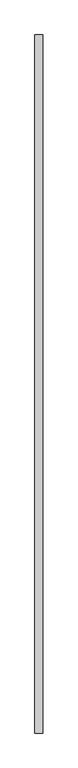
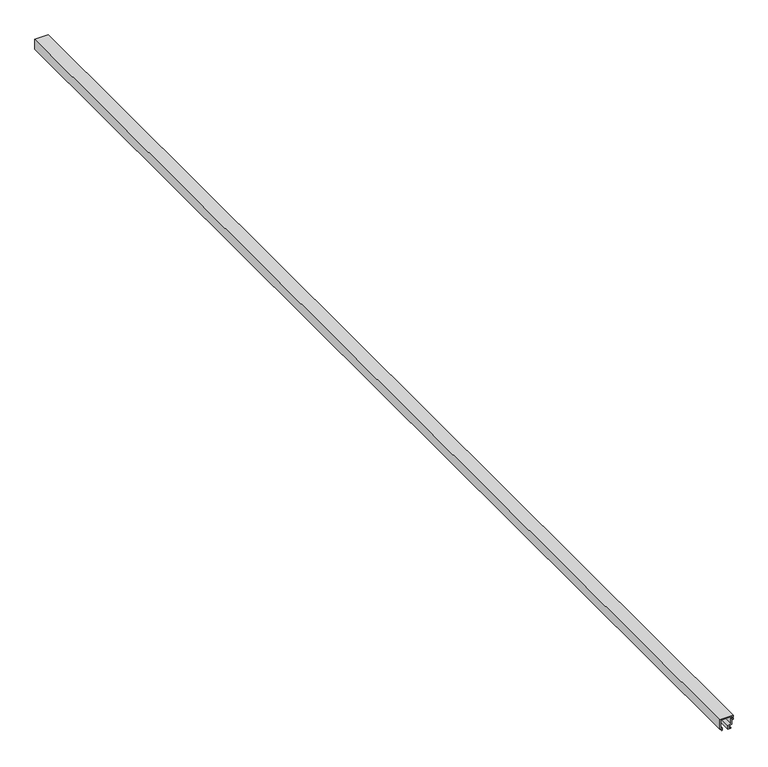
"""IFC4 building model written with IfcOpenShell, lengths in millimetres: proxy geometry, Door frame8:Door frame008:296226 : Door frame8:Door frame008:296226."""

from ifc_helpers import new_model, si_unit, frame, origin, place, context, project, spatial, polyline, outline, extrude, source, transform, mapped, element, save


def generic_models_a8a23339(model_context):
    return source(origin(), model_context, "Body", "SweptSolid", [
        extrude(outline(polyline([(36671.1866406, 20295.6019553), (36665.0550947, 20295.6019553), (36665.0550947, 20300.3039019), (36666.4520947, 20300.3039019), (36666.4520947, 20297.1767553), (36670.1011414, 20297.1767553), (36671.9000345, 20301.9015595), (36679.2790947, 20301.9015595), (36679.2790947, 20304.4415595), (36681.9249044, 20304.4415595), (36681.9249044, 20303.1868839), (36680.6298938, 20303.1868839), (36680.6298938, 20301.7018641), (36685.5545864, 20301.7018641), (36685.5545864, 20303.1868839), (36684.2230088, 20303.1868839), (36684.2230088, 20304.4415595), (36686.8990947, 20304.4415595), (36686.8990947, 20281.8355595), (36669.5427612, 20281.8355595), (36669.5427612, 20284.7819595), (36668.8374665, 20285.1817657), (36667.4225662, 20284.3648726), (36666.0872218, 20285.7002171), (36666.4062067, 20286.5599595), (36670.8462947, 20286.5599595), (36670.8462947, 20283.2325595), (36685.5020947, 20283.2325595), (36685.5020947, 20300.5045595), (36673.0532282, 20300.5045595), (36671.1866406, 20295.6019553)])), frame((0.0, -774.5581156, 0.0), z_axis=(0.0, 1.0, 0.0), x_axis=(0.0, 0.0, 1.0)), (0.0, 0.0, 1.0), 1999.85),
    ])


if __name__ == "__main__":
    model = new_model("IFC4")
    model_context = context("Model", 3, world=origin())
    ifc_project = project(units=[si_unit("LENGTHUNIT", "METRE", prefix="MILLI")], contexts=[model_context])
    site = spatial("IfcSite", under=ifc_project)
    building = spatial("IfcBuilding", under=site)
    placement = place(None, origin())
    generic_models_shape = generic_models_a8a23339(model_context)
    element("IfcBuildingElementProxy", 1, Name="Door frame8:Door frame008:296226 : Door frame8:Door frame008:296226", ObjectType="Door frame8:Door frame008:296226 : Door frame8:Door frame008:296226", at=placement, inside=building, context=model_context, shape_type="MappedRepresentation", body=[
        mapped(generic_models_shape, transform((0.0, 0.0, 0.0), x_axis=(1.0, 0.0, 0.0), y_axis=(0.0, 1.0, 0.0), z_axis=(0.0, 0.0, 1.0))),
    ])
    save(model, "model.ifc")

# Revit data of these elements
# Type "Door frame8:Door frame008:296226 : Door frame8:Door frame008:296226"
#   NameOverride = "Door frame8:Door frame008:296226"
#   ObjectTypeOverride = "Door frame8:Door frame008"
#   Reference = "Door frame008"
#   Category = "Generic Models"
#   Tag = "296226"
# Element 1 (IfcBuildingElementProxy, "Door frame8:Door frame008:296226 : Door frame8:Door frame008:296226")
#   Materials on its faces: "FLEETWOOD SERIES T-3200 SINGLE SWING DOOR FRAME"
# Materials
#   "FLEETWOOD SERIES T-3200 SINGLE SWING DOOR FRAME": class "Unassigned", colour RGB 128 128 128, transparency 0, Cost = 0
